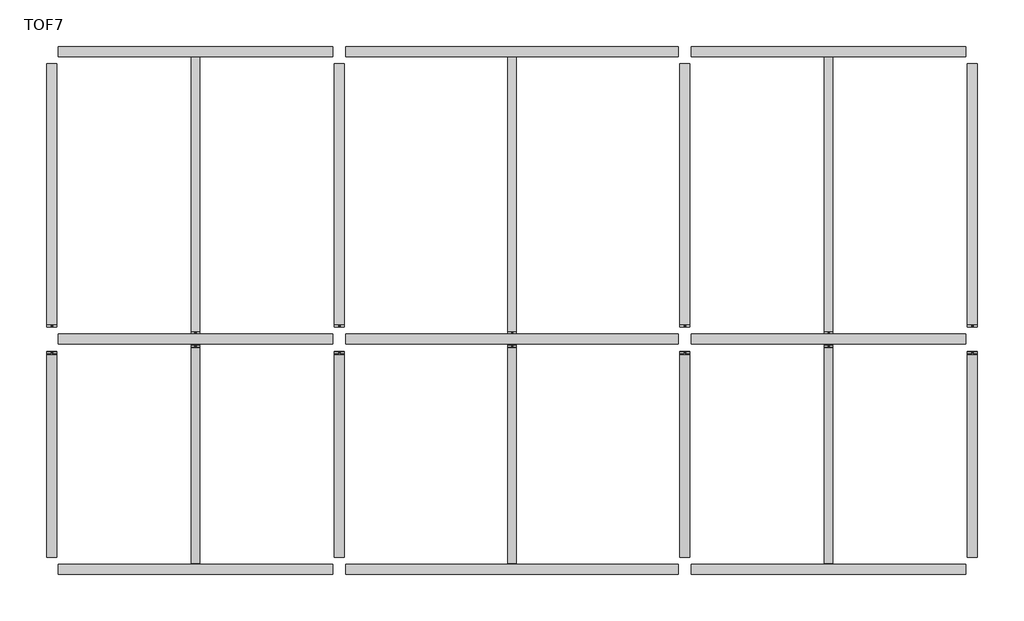
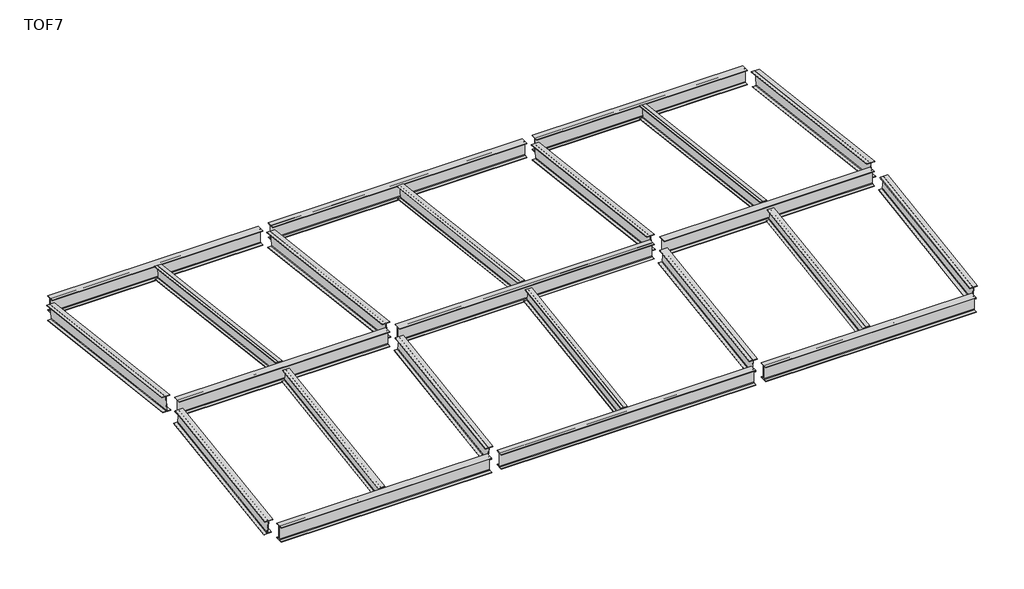
# One storey: 23 beams.
"""IFC4 building model written with IfcOpenShell, lengths in millimetres."""

import ifcopenshell
import ifcopenshell.guid

model = None  # the IFC model being written
_history = None  # IfcOwnerHistory: only IFC2X3 demands one
_inside = {}  # id of a spatial element -> (the spatial element, [elements in it])
_under = {}  # id of a project, library or spatial element -> (it, [spatial elements below it])
_declared = {}  # id of a project -> (the project, [libraries it declares])
_typed = {}  # id of a type object -> (the type object, [elements of that type])
_made_of = {}  # id of a material, layer set ... -> (it, [elements and type objects made of it])


def new_model(schema):
    """Start an empty IFC model of exactly this schema.

    Asked for "IFC4X3", IfcOpenShell would pick the latest addendum, in which some entities
    have other attributes; the version numbers below select the first issue.
    IFC2X3 requires an IfcOwnerHistory on every rooted entity: one is made here for all.
    """
    global model, _history
    if schema == "IFC4X3":
        model = ifcopenshell.file(schema_version=(4, 3, 0, 0))
    else:
        model = ifcopenshell.file(schema=schema)
    _inside.clear()
    _under.clear()
    _declared.clear()
    _typed.clear()
    _made_of.clear()
    _history = None
    if model.schema == "IFC2X3":
        org = make("IfcOrganization", Name="unknown")
        user = make(
            "IfcPersonAndOrganization",
            ThePerson=make("IfcPerson", FamilyName="unknown"),
            TheOrganization=org,
        )
        app = make(
            "IfcApplication",
            ApplicationDeveloper=org,
            Version="unknown",
            ApplicationFullName="unknown",
            ApplicationIdentifier="unknown",
        )
        _history = make(
            "IfcOwnerHistory",
            OwningUser=user,
            OwningApplication=app,
            ChangeAction="ADDED",
            CreationDate=0,
        )
    return model


def make(cls, **values):
    """One entity of the class cls with the attributes given. An attribute that is None is left unset."""
    return model.create_entity(
        cls, **{name: value for name, value in values.items() if value is not None}
    )


def rooted(cls, **values):
    """An entity with a GlobalId (a new one), such as an element, a storey or a relation."""
    return make(cls, GlobalId=ifcopenshell.guid.new(), OwnerHistory=_history, **values)


def si_unit(unit_type, name, prefix=None):
    """IfcSIUnit, for example si_unit("LENGTHUNIT", "METRE", prefix="MILLI")."""
    return make("IfcSIUnit", UnitType=unit_type, Prefix=prefix, Name=name)


def assignment(units):
    """IfcUnitAssignment: the units of a project."""
    return None if units is None else make("IfcUnitAssignment", Units=units)


def point(xyz):
    """IfcCartesianPoint."""
    return None if xyz is None else make("IfcCartesianPoint", Coordinates=xyz)


def direction(xyz):
    """IfcDirection."""
    return None if xyz is None else make("IfcDirection", DirectionRatios=xyz)


def frame(location, z_axis=None, x_axis=None):
    """IfcAxis2Placement3D, a coordinate frame: its origin and axes. An axis left out is left unset."""
    return make(
        "IfcAxis2Placement3D",
        Location=point(location),
        Axis=direction(z_axis),
        RefDirection=direction(x_axis),
    )


def frame_2d(location, x_axis=None):
    """IfcAxis2Placement2D, a coordinate frame in the plane: its origin and x axis."""
    return make(
        "IfcAxis2Placement2D", Location=point(location), RefDirection=direction(x_axis)
    )


def origin():
    """The frame at (0, 0, 0) with its axes left unset."""
    return frame((0.0, 0.0, 0.0))


def place(relative_to, where):
    """IfcLocalPlacement: puts the frame where relative to a parent placement (None: the world)."""
    return make(
        "IfcLocalPlacement", PlacementRelTo=relative_to, RelativePlacement=where
    )


def context(
    kind, dimensions, precision=None, world=None, true_north=None, identifier=None
):
    """IfcGeometricRepresentationContext, for example the 3D "Model" context."""
    return make(
        "IfcGeometricRepresentationContext",
        ContextIdentifier=identifier,
        ContextType=kind,
        CoordinateSpaceDimension=dimensions,
        Precision=precision,
        WorldCoordinateSystem=world,
        TrueNorth=true_north,
    )


def project(units=None, contexts=None):
    """IfcProject with its units and contexts."""
    return rooted(
        "IfcProject",
        Name="project",
        RepresentationContexts=contexts,
        UnitsInContext=assignment(units),
    )


def spatial(cls, under=None, at=None, **own):
    """A site, building, storey or space (cls), placed at a placement, below another one or the project."""
    s = rooted(cls, ObjectPlacement=at, **own)
    if under is not None:
        _under.setdefault(under.id(), (under, []))[1].append(s)
    return s


def polyline(points):
    """IfcPolyline through the points."""
    return make("IfcPolyline", Points=[point(p) for p in points])


def circle_curve(where, radius):
    """IfcCircle in the frame where."""
    return make("IfcCircle", Position=where, Radius=radius)


def trimmed(basis, trim1, trim2, sense, master):
    """IfcTrimmedCurve: the piece of a basis curve between two trims."""
    return make(
        "IfcTrimmedCurve",
        BasisCurve=basis,
        Trim1=trim1,
        Trim2=trim2,
        SenseAgreement=sense,
        MasterRepresentation=master,
    )


def segment(curve, same_sense, transition):
    """IfcCompositeCurveSegment."""
    return make(
        "IfcCompositeCurveSegment",
        Transition=transition,
        SameSense=same_sense,
        ParentCurve=curve,
    )


def composite_curve(segments, self_intersect=None):
    """IfcCompositeCurve: segments joined end to end."""
    return make("IfcCompositeCurve", Segments=segments, SelfIntersect=self_intersect)


def outline(outer, holes=None, kind="AREA"):
    """IfcArbitraryClosedProfileDef: a profile drawn as a closed curve; with holes, ...WithVoids."""
    if holes is None:
        return make("IfcArbitraryClosedProfileDef", ProfileType=kind, OuterCurve=outer)
    return make(
        "IfcArbitraryProfileDefWithVoids",
        ProfileType=kind,
        OuterCurve=outer,
        InnerCurves=holes,
    )


def extrude(swept, where, along, depth):
    """IfcExtrudedAreaSolid: the profile swept, set in the frame where, extruded along a direction by depth."""
    return make(
        "IfcExtrudedAreaSolid",
        SweptArea=swept,
        Position=where,
        ExtrudedDirection=direction(along),
        Depth=depth,
    )


def shape(context_of_items, identifier, shape_type, items):
    """IfcShapeRepresentation: the items that make up one representation, for example the "Body"."""
    return make(
        "IfcShapeRepresentation",
        ContextOfItems=context_of_items,
        RepresentationIdentifier=identifier,
        RepresentationType=shape_type,
        Items=items,
    )


def source(mapping_origin, context_of_items, identifier, shape_type, items):
    """IfcRepresentationMap: a shape defined once, which mapped items show again and again."""
    return make(
        "IfcRepresentationMap",
        MappingOrigin=mapping_origin,
        MappedRepresentation=shape(context_of_items, identifier, shape_type, items),
    )


def transform(
    local_origin,
    x_axis=None,
    y_axis=None,
    z_axis=None,
    scale=None,
    scale2=None,
    scale3=None,
    uniform=True,
):
    """IfcCartesianTransformationOperator3D, or its non-uniform kind. x_axis, y_axis, z_axis: its Axis1, 2, 3."""
    if uniform:
        return make(
            "IfcCartesianTransformationOperator3D",
            Axis1=direction(x_axis),
            Axis2=direction(y_axis),
            LocalOrigin=point(local_origin),
            Scale=scale,
            Axis3=direction(z_axis),
        )
    return make(
        "IfcCartesianTransformationOperator3DnonUniform",
        Axis1=direction(x_axis),
        Axis2=direction(y_axis),
        LocalOrigin=point(local_origin),
        Scale=scale,
        Axis3=direction(z_axis),
        Scale2=scale2,
        Scale3=scale3,
    )


def mapped(mapping_source, mapping_target):
    """IfcMappedItem: shows the shape of a source again, moved by a transform."""
    return make(
        "IfcMappedItem", MappingSource=mapping_source, MappingTarget=mapping_target
    )


def made_of(thing, what):
    """Note that an element or type object is made of a material, layer set ...; save() writes the relation."""
    if what is not None:
        _made_of.setdefault(what.id(), (what, []))[1].append(thing)
    return thing


def element(
    cls,
    number,
    at=None,
    inside=None,
    cuts=None,
    type_object=None,
    material=None,
    context=None,
    identifier="Body",
    shape_type=None,
    held_by="IfcProductDefinitionShape",
    body=None,
    shapes=None,
    **own,
):
    """One element of the class cls, such as IfcWall. Its Tag is "e" and its number.

    at: its placement. inside: the storey or other place that contains it. cuts: it is an
    opening in that element (IfcRelVoidsElement). A single representation is given by context,
    identifier, shape_type and body (its items); several are given by shapes. held_by: the class
    of the entity that holds the representations. save() writes the other relations.
    """
    e = rooted(cls, Tag="e%d" % number, ObjectPlacement=at, **own)
    if body is not None:
        shapes = [shape(context, identifier, shape_type, body)]
    if shapes is not None:
        e.Representation = make(held_by, Representations=shapes)
    if inside is not None:
        _inside.setdefault(inside.id(), (inside, []))[1].append(e)
    if cuts is not None:
        rooted(
            "IfcRelVoidsElement", RelatingBuildingElement=cuts, RelatedOpeningElement=e
        )
    if type_object is not None:
        _typed.setdefault(type_object.id(), (type_object, []))[1].append(e)
    return made_of(e, material)


def aggregate(whole, parts):
    """IfcRelAggregates: a whole, such as a stair, and the parts it consists of."""
    return rooted("IfcRelAggregates", RelatingObject=whole, RelatedObjects=parts)


def save(model, path):
    """Write the relations noted so far, then the file.

    IfcRelAggregates (storeys below a building ...), IfcRelContainedInSpatialStructure (elements
    in a storey), IfcRelDefinesByType, IfcRelAssociatesMaterial and IfcRelDeclares: one each for
    every whole, place, type object, material and project.
    """
    for whole, parts in _under.values():
        aggregate(whole, parts)
    for where, things in _inside.values():
        rooted(
            "IfcRelContainedInSpatialStructure",
            RelatedElements=things,
            RelatingStructure=where,
        )
    for kind, things in _typed.values():
        rooted("IfcRelDefinesByType", RelatedObjects=things, RelatingType=kind)
    for what, things in _made_of.values():
        rooted("IfcRelAssociatesMaterial", RelatedObjects=things, RelatingMaterial=what)
    for by, libraries in _declared.values():
        rooted("IfcRelDeclares", RelatingContext=by, RelatedDefinitions=libraries)
    model.write(path)


def beam_c38fbaf3(model_context):
    return source(origin(), model_context, "Body", "SweptSolid", [
        extrude(outline(composite_curve([segment(polyline([(75.0, -141.0), (75.0, -150.0), (-75.0, -150.0), (-75.0, -141.0), (-16.25, -141.0)]), True, "CONTINUOUS"), segment(trimmed(circle_curve(frame_2d((-16.25, -128.0)), 13.0), [point((-16.25, -141.0))], [point((-3.25, -128.0))], True, "CARTESIAN"), True, "CONTINUOUS"), segment(polyline([(-3.25, -128.0), (-3.25, 128.0)]), True, "CONTINUOUS"), segment(trimmed(circle_curve(frame_2d((-16.25, 128.0)), 13.0), [point((-3.25, 128.0))], [point((-16.25, 141.0))], True, "CARTESIAN"), True, "CONTINUOUS"), segment(polyline([(-16.25, 141.0), (-75.0, 141.0), (-75.0, 150.0), (75.0, 150.0), (75.0, 141.0), (16.25, 141.0)]), True, "CONTINUOUS"), segment(trimmed(circle_curve(frame_2d((16.25, 128.0)), 13.0), [point((16.25, 141.0))], [point((3.25, 128.0))], True, "CARTESIAN"), True, "CONTINUOUS"), segment(polyline([(3.25, 128.0), (3.25, -128.0)]), True, "CONTINUOUS"), segment(trimmed(circle_curve(frame_2d((16.25, -128.0)), 13.0), [point((3.25, -128.0))], [point((16.25, -141.0))], True, "CARTESIAN"), True, "CONTINUOUS"), segment(polyline([(16.25, -141.0), (75.0, -141.0)]), True, "CONTINUOUS")], self_intersect=False)), frame((-1923.1429107, 0.0, 0.0), z_axis=(1.0, 0.0, 0.0), x_axis=(0.0, 1.0, 0.0)), (0.0, 0.0, 1.0), 3799.338853),
    ])


def beam_fed367b4(model_context):
    return source(origin(), model_context, "Body", "SweptSolid", [
        extrude(outline(composite_curve([segment(polyline([(75.0, -141.0), (75.0, -150.0), (-75.0, -150.0), (-75.0, -141.0), (-16.25, -141.0)]), True, "CONTINUOUS"), segment(trimmed(circle_curve(frame_2d((-16.25, -128.0)), 13.0), [point((-16.25, -141.0))], [point((-3.25, -128.0))], True, "CARTESIAN"), True, "CONTINUOUS"), segment(polyline([(-3.25, -128.0), (-3.25, 128.0)]), True, "CONTINUOUS"), segment(trimmed(circle_curve(frame_2d((-16.25, 128.0)), 13.0), [point((-3.25, 128.0))], [point((-16.25, 141.0))], True, "CARTESIAN"), True, "CONTINUOUS"), segment(polyline([(-16.25, 141.0), (-75.0, 141.0), (-75.0, 150.0), (75.0, 150.0), (75.0, 141.0), (16.25, 141.0)]), True, "CONTINUOUS"), segment(trimmed(circle_curve(frame_2d((16.25, 128.0)), 13.0), [point((16.25, 141.0))], [point((3.25, 128.0))], True, "CARTESIAN"), True, "CONTINUOUS"), segment(polyline([(3.25, 128.0), (3.25, -128.0)]), True, "CONTINUOUS"), segment(trimmed(circle_curve(frame_2d((16.25, -128.0)), 13.0), [point((3.25, -128.0))], [point((16.25, -141.0))], True, "CARTESIAN"), True, "CONTINUOUS"), segment(polyline([(16.25, -141.0), (75.0, -141.0)]), True, "CONTINUOUS")], self_intersect=False)), frame((-2381.1079142, 0.0, 0.0), z_axis=(1.0, 0.0, 0.0), x_axis=(0.0, 1.0, 0.0)), (0.0, 0.0, 1.0), 4799.4668533),
    ])


def beam_74d50635(model_context):
    return source(origin(), model_context, "Body", "SweptSolid", [
        extrude(outline(composite_curve([segment(polyline([(87.5, -164.0), (87.5, -175.0), (-87.5, -175.0), (-87.5, -164.0), (-17.5, -164.0)]), True, "CONTINUOUS"), segment(trimmed(circle_curve(frame_2d((-17.5, -150.0)), 14.0), [point((-17.5, -164.0))], [point((-3.5, -150.0))], True, "CARTESIAN"), True, "CONTINUOUS"), segment(polyline([(-3.5, -150.0), (-3.5, 150.0)]), True, "CONTINUOUS"), segment(trimmed(circle_curve(frame_2d((-17.5, 150.0)), 14.0), [point((-3.5, 150.0))], [point((-17.5, 164.0))], True, "CARTESIAN"), True, "CONTINUOUS"), segment(polyline([(-17.5, 164.0), (-87.5, 164.0), (-87.5, 175.0), (87.5, 175.0), (87.5, 164.0), (17.5, 164.0)]), True, "CONTINUOUS"), segment(trimmed(circle_curve(frame_2d((17.5, 150.0)), 14.0), [point((17.5, 164.0))], [point((3.5, 150.0))], True, "CARTESIAN"), True, "CONTINUOUS"), segment(polyline([(3.5, 150.0), (3.5, -150.0)]), True, "CONTINUOUS"), segment(trimmed(circle_curve(frame_2d((17.5, -150.0)), 14.0), [point((3.5, -150.0))], [point((17.5, -164.0))], True, "CARTESIAN"), True, "CONTINUOUS"), segment(polyline([(17.5, -164.0), (87.5, -164.0)]), True, "CONTINUOUS")], self_intersect=False)), frame((-2387.3, 0.0, 0.0), z_axis=(1.0, 0.0, 0.0), x_axis=(0.0, 1.0, 0.0)), (0.0, 0.0, 1.0), 4774.6),
    ])


def beam_3a5a8fac(model_context):
    return source(origin(), model_context, "Body", "SweptSolid", [
        extrude(outline(composite_curve([segment(polyline([(87.5, -164.0), (87.5, -175.0), (-87.5, -175.0), (-87.5, -164.0), (-17.5, -164.0)]), True, "CONTINUOUS"), segment(trimmed(circle_curve(frame_2d((-17.5, -150.0)), 14.0), [point((-17.5, -164.0))], [point((-3.5, -150.0))], True, "CARTESIAN"), True, "CONTINUOUS"), segment(polyline([(-3.5, -150.0), (-3.5, 150.0)]), True, "CONTINUOUS"), segment(trimmed(circle_curve(frame_2d((-17.5, 150.0)), 14.0), [point((-3.5, 150.0))], [point((-17.5, 164.0))], True, "CARTESIAN"), True, "CONTINUOUS"), segment(polyline([(-17.5, 164.0), (-87.5, 164.0), (-87.5, 175.0), (87.5, 175.0), (87.5, 164.0), (17.5, 164.0)]), True, "CONTINUOUS"), segment(trimmed(circle_curve(frame_2d((17.5, 150.0)), 14.0), [point((17.5, 164.0))], [point((3.5, 150.0))], True, "CARTESIAN"), True, "CONTINUOUS"), segment(polyline([(3.5, 150.0), (3.5, -150.0)]), True, "CONTINUOUS"), segment(trimmed(circle_curve(frame_2d((17.5, -150.0)), 14.0), [point((3.5, -150.0))], [point((17.5, -164.0))], True, "CARTESIAN"), True, "CONTINUOUS"), segment(polyline([(17.5, -164.0), (87.5, -164.0)]), True, "CONTINUOUS")], self_intersect=False)), frame((-2887.3, 0.0, 0.0), z_axis=(1.0, 0.0, 0.0), x_axis=(0.0, 1.0, 0.0)), (0.0, 0.0, 1.0), 5774.6),
    ])


def beam_9c24ba7d(model_context):
    return source(origin(), model_context, "Body", "SweptSolid", [
        extrude(outline(composite_curve([segment(polyline([(87.5, -164.0), (87.5, -175.0), (-87.5, -175.0), (-87.5, -164.0), (-17.5, -164.0)]), True, "CONTINUOUS"), segment(trimmed(circle_curve(frame_2d((-17.5, -150.0)), 14.0), [point((-17.5, -164.0))], [point((-3.5, -150.0))], True, "CARTESIAN"), True, "CONTINUOUS"), segment(polyline([(-3.5, -150.0), (-3.5, 150.0)]), True, "CONTINUOUS"), segment(trimmed(circle_curve(frame_2d((-17.5, 150.0)), 14.0), [point((-3.5, 150.0))], [point((-17.5, 164.0))], True, "CARTESIAN"), True, "CONTINUOUS"), segment(polyline([(-17.5, 164.0), (-87.5, 164.0), (-87.5, 175.0), (87.5, 175.0), (87.5, 164.0), (17.5, 164.0)]), True, "CONTINUOUS"), segment(trimmed(circle_curve(frame_2d((17.5, 150.0)), 14.0), [point((17.5, 164.0))], [point((3.5, 150.0))], True, "CARTESIAN"), True, "CONTINUOUS"), segment(polyline([(3.5, 150.0), (3.5, -150.0)]), True, "CONTINUOUS"), segment(trimmed(circle_curve(frame_2d((17.5, -150.0)), 14.0), [point((3.5, -150.0))], [point((17.5, -164.0))], True, "CARTESIAN"), True, "CONTINUOUS"), segment(polyline([(17.5, -164.0), (87.5, -164.0)]), True, "CONTINUOUS")], self_intersect=False)), frame((-1811.887571, 0.0, 0.0), z_axis=(1.0, 0.0, 0.0), x_axis=(0.0, 1.0, 0.0)), (0.0, 0.0, 1.0), 3566.8249285),
    ])


def beam_94df1702(model_context):
    return source(origin(), model_context, "Body", "SweptSolid", [
        extrude(outline(composite_curve([segment(polyline([(87.5, -164.0), (87.5, -175.0), (-87.5, -175.0), (-87.5, -164.0), (-17.5, -164.0)]), True, "CONTINUOUS"), segment(trimmed(circle_curve(frame_2d((-17.5, -150.0)), 14.0), [point((-17.5, -164.0))], [point((-3.5, -150.0))], True, "CARTESIAN"), True, "CONTINUOUS"), segment(polyline([(-3.5, -150.0), (-3.5, 150.0)]), True, "CONTINUOUS"), segment(trimmed(circle_curve(frame_2d((-17.5, 150.0)), 14.0), [point((-3.5, 150.0))], [point((-17.5, 164.0))], True, "CARTESIAN"), True, "CONTINUOUS"), segment(polyline([(-17.5, 164.0), (-87.5, 164.0), (-87.5, 175.0), (87.5, 175.0), (87.5, 164.0), (17.5, 164.0)]), True, "CONTINUOUS"), segment(trimmed(circle_curve(frame_2d((17.5, 150.0)), 14.0), [point((17.5, 164.0))], [point((3.5, 150.0))], True, "CARTESIAN"), True, "CONTINUOUS"), segment(polyline([(3.5, 150.0), (3.5, -150.0)]), True, "CONTINUOUS"), segment(trimmed(circle_curve(frame_2d((17.5, -150.0)), 14.0), [point((3.5, -150.0))], [point((17.5, -164.0))], True, "CARTESIAN"), True, "CONTINUOUS"), segment(polyline([(17.5, -164.0), (87.5, -164.0)]), True, "CONTINUOUS")], self_intersect=False)), frame((-2261.8008094, 0.0, 0.0), z_axis=(1.0, 0.0, 0.0), x_axis=(0.0, 1.0, 0.0)), (0.0, 0.0, 1.0), 4568.4611041),
    ])


model = new_model("IFC4")

# Units and contexts
model_context = context("Model", 3, world=origin())
ifc_project = project(units=[si_unit("LENGTHUNIT", "METRE", prefix="MILLI")], contexts=[model_context])

# Site, building, storey
site = spatial("IfcSite", under=ifc_project)
building = spatial("IfcBuilding", under=site)
storey = spatial("IfcBuildingStorey", under=building, Name="TOF7", Elevation=12500.0)

# Beams
placement = place(None, origin())
beam_shape = beam_c38fbaf3(model_context)
element("IfcBeam", 1, ObjectType="0912_Steel Framing_H-KSD3502 : H_SB_AR_S02_H-300x150x6.5x9_Stair", at=placement, inside=storey, context=model_context, shape_type="MappedRepresentation", body=[
    mapped(beam_shape, transform((2500.0, 2022.2510679, 12651.6595471), x_axis=(0.0, 0.9889363528682974, 0.14834045293024514), y_axis=(-1.0, 0.0, 0.0), z_axis=(0.0, -0.14834045293024517, 0.9889363528682975))),
])
element("IfcBeam", 2, ObjectType="0912_Steel Framing_H-KSD3502 : H_SB_AR_S02_H-300x150x6.5x9_Stair", at=placement, inside=storey, context=model_context, shape_type="MappedRepresentation", body=[
    mapped(beam_shape, transform((8000.0, 2022.2510679, 12651.6595471), x_axis=(0.0, 0.9889363528682974, 0.14834045293024514), y_axis=(-1.0, 0.0, 0.0), z_axis=(0.0, -0.14834045293024517, 0.9889363528682975))),
])
element("IfcBeam", 3, ObjectType="0912_Steel Framing_H-KSD3502 : H_SB_AR_S02_H-300x150x6.5x9_Stair", at=placement, inside=storey, context=model_context, shape_type="MappedRepresentation", body=[
    mapped(beam_shape, transform((13500.0, 2022.2510679, 12651.6595471), x_axis=(0.0, 0.9889363528682974, 0.14834045293024514), y_axis=(-1.0, 0.0, 0.0), z_axis=(0.0, -0.14834045293024517, 0.9889363528682975))),
])
beam_2_shape = beam_fed367b4(model_context)
element("IfcBeam", 4, ObjectType="0912_Steel Framing_H-KSD3502 : H_SB_AR_S02_H-300x150x6.5x9_Stair", at=placement, inside=storey, context=model_context, shape_type="MappedRepresentation", body=[
    mapped(beam_2_shape, transform((2500.0, 6482.1282169, 12651.0684742), x_axis=(0.0, 0.992876838486922, -0.11914522061843061), y_axis=(-1.0, 0.0, 0.0), z_axis=(0.0, 0.11914522061843062, 0.9928768384869221))),
])
element("IfcBeam", 5, ObjectType="0912_Steel Framing_H-KSD3502 : H_SB_AR_S02_H-300x150x6.5x9_Stair", at=placement, inside=storey, context=model_context, shape_type="MappedRepresentation", body=[
    mapped(beam_2_shape, transform((8000.0, 6482.1282169, 12651.0684742), x_axis=(0.0, 0.992876838486922, -0.11914522061843061), y_axis=(-1.0, 0.0, 0.0), z_axis=(0.0, 0.11914522061843062, 0.9928768384869221))),
])
element("IfcBeam", 6, ObjectType="0912_Steel Framing_H-KSD3502 : H_SB_AR_S02_H-300x150x6.5x9_Stair", at=placement, inside=storey, context=model_context, shape_type="MappedRepresentation", body=[
    mapped(beam_2_shape, transform((13500.0, 6482.1282169, 12651.0684742), x_axis=(0.0, 0.992876838486922, -0.11914522061843061), y_axis=(-1.0, 0.0, 0.0), z_axis=(0.0, 0.11914522061843062, 0.9928768384869221))),
])
beam_3_shape = beam_74d50635(model_context)
element("IfcBeam", 7, ObjectType="0912_Steel Framing_H-KSD3502 : H_SB_AR_S02_H-350x175x7x11_Platform", at=placement, inside=storey, context=model_context, shape_type="MappedRepresentation", body=[
    mapped(beam_3_shape, transform((2500.0, 0.0, 12325.0), x_axis=(1.0, 0.0, 0.0), y_axis=(0.0, 1.0, 0.0), z_axis=(0.0, 0.0, 1.0))),
])
element("IfcBeam", 8, ObjectType="0912_Steel Framing_H-KSD3502 : H_SB_AR_S02_H-350x175x7x11_Platform", at=placement, inside=storey, context=model_context, shape_type="MappedRepresentation", body=[
    mapped(beam_3_shape, transform((13500.0, 0.0, 12325.0), x_axis=(1.0, 0.0, 0.0), y_axis=(0.0, 1.0, 0.0), z_axis=(0.0, 0.0, 1.0))),
])
element("IfcBeam", 9, ObjectType="0912_Steel Framing_H-KSD3502 : H_SB_AR_S02_H-350x175x7x11_Platform", at=placement, inside=storey, context=model_context, shape_type="MappedRepresentation", body=[
    mapped(beam_3_shape, transform((2500.0, 4000.0, 12925.0), x_axis=(1.0, 0.0, 0.0), y_axis=(0.0, 1.0, 0.0), z_axis=(0.0, 0.0, 1.0))),
])
element("IfcBeam", 10, ObjectType="0912_Steel Framing_H-KSD3502 : H_SB_AR_S02_H-350x175x7x11_Platform", at=placement, inside=storey, context=model_context, shape_type="MappedRepresentation", body=[
    mapped(beam_3_shape, transform((13500.0, 4000.0, 12925.0), x_axis=(1.0, 0.0, 0.0), y_axis=(0.0, 1.0, 0.0), z_axis=(0.0, 0.0, 1.0))),
])
element("IfcBeam", 11, ObjectType="0912_Steel Framing_H-KSD3502 : H_SB_AR_S02_H-350x175x7x11_Platform", at=placement, inside=storey, context=model_context, shape_type="MappedRepresentation", body=[
    mapped(beam_3_shape, transform((2500.0, 9000.0, 12325.0), x_axis=(1.0, 0.0, 0.0), y_axis=(0.0, 1.0, 0.0), z_axis=(0.0, 0.0, 1.0))),
])
element("IfcBeam", 12, ObjectType="0912_Steel Framing_H-KSD3502 : H_SB_AR_S02_H-350x175x7x11_Platform", at=placement, inside=storey, context=model_context, shape_type="MappedRepresentation", body=[
    mapped(beam_3_shape, transform((13500.0, 9000.0, 12325.0), x_axis=(1.0, 0.0, 0.0), y_axis=(0.0, 1.0, 0.0), z_axis=(0.0, 0.0, 1.0))),
])
beam_4_shape = beam_3a5a8fac(model_context)
element("IfcBeam", 13, ObjectType="0912_Steel Framing_H-KSD3502 : H_SB_AR_S02_H-350x175x7x11_Platform", at=placement, inside=storey, context=model_context, shape_type="MappedRepresentation", body=[
    mapped(beam_4_shape, transform((8000.0, 0.0, 12325.0), x_axis=(1.0, 0.0, 0.0), y_axis=(0.0, 1.0, 0.0), z_axis=(0.0, 0.0, 1.0))),
])
element("IfcBeam", 14, ObjectType="0912_Steel Framing_H-KSD3502 : H_SB_AR_S02_H-350x175x7x11_Platform", at=placement, inside=storey, context=model_context, shape_type="MappedRepresentation", body=[
    mapped(beam_4_shape, transform((8000.0, 4000.0, 12925.0), x_axis=(1.0, 0.0, 0.0), y_axis=(0.0, 1.0, 0.0), z_axis=(0.0, 0.0, 1.0))),
])
element("IfcBeam", 15, ObjectType="0912_Steel Framing_H-KSD3502 : H_SB_AR_S02_H-350x175x7x11_Platform", at=placement, inside=storey, context=model_context, shape_type="MappedRepresentation", body=[
    mapped(beam_4_shape, transform((8000.0, 9000.0, 12325.0), x_axis=(1.0, 0.0, 0.0), y_axis=(0.0, 1.0, 0.0), z_axis=(0.0, 0.0, 1.0))),
])
beam_5_shape = beam_9c24ba7d(model_context)
element("IfcBeam", 16, ObjectType="0912_Steel Framing_H-KSD3502 : H_SB_AR_S02_H-350x175x7x11_Platform", at=placement, inside=storey, context=model_context, shape_type="MappedRepresentation", body=[
    mapped(beam_5_shape, transform((0.0, 2025.9595793, 12626.9361382), x_axis=(0.0, 0.9889363528682974, 0.14834045293024514), y_axis=(-1.0, 0.0, 0.0), z_axis=(0.0, -0.14834045293024517, 0.9889363528682975))),
])
element("IfcBeam", 17, ObjectType="0912_Steel Framing_H-KSD3502 : H_SB_AR_S02_H-350x175x7x11_Platform", at=placement, inside=storey, context=model_context, shape_type="MappedRepresentation", body=[
    mapped(beam_5_shape, transform((5000.0, 2025.9595793, 12626.9361382), x_axis=(0.0, 0.9889363528682974, 0.14834045293024514), y_axis=(-1.0, 0.0, 0.0), z_axis=(0.0, -0.14834045293024517, 0.9889363528682975))),
])
element("IfcBeam", 18, ObjectType="0912_Steel Framing_H-KSD3502 : H_SB_AR_S02_H-350x175x7x11_Platform", at=placement, inside=storey, context=model_context, shape_type="MappedRepresentation", body=[
    mapped(beam_5_shape, transform((11000.0, 2025.9595793, 12626.9361382), x_axis=(0.0, 0.9889363528682974, 0.14834045293024514), y_axis=(-1.0, 0.0, 0.0), z_axis=(0.0, -0.14834045293024517, 0.9889363528682975))),
])
element("IfcBeam", 19, ObjectType="0912_Steel Framing_H-KSD3502 : H_SB_AR_S02_H-350x175x7x11_Platform", at=placement, inside=storey, context=model_context, shape_type="MappedRepresentation", body=[
    mapped(beam_5_shape, transform((16000.0, 2025.9595793, 12626.9361382), x_axis=(0.0, 0.9889363528682974, 0.14834045293024514), y_axis=(-1.0, 0.0, 0.0), z_axis=(0.0, -0.14834045293024517, 0.9889363528682975))),
])
beam_6_shape = beam_94df1702(model_context)
element("IfcBeam", 20, ObjectType="0912_Steel Framing_H-KSD3502 : H_SB_AR_S02_H-350x175x7x11_Platform", at=placement, inside=storey, context=model_context, shape_type="MappedRepresentation", body=[
    mapped(beam_6_shape, transform((0.0, 6479.1495864, 12626.2465533), x_axis=(0.0, 0.992876838486922, -0.11914522061843061), y_axis=(-1.0, 0.0, 0.0), z_axis=(0.0, 0.11914522061843065, 0.9928768384869221))),
])
element("IfcBeam", 21, ObjectType="0912_Steel Framing_H-KSD3502 : H_SB_AR_S02_H-350x175x7x11_Platform", at=placement, inside=storey, context=model_context, shape_type="MappedRepresentation", body=[
    mapped(beam_6_shape, transform((5000.0, 6479.1495864, 12626.2465533), x_axis=(0.0, 0.992876838486922, -0.11914522061843061), y_axis=(-1.0, 0.0, 0.0), z_axis=(0.0, 0.11914522061843065, 0.9928768384869221))),
])
element("IfcBeam", 22, ObjectType="0912_Steel Framing_H-KSD3502 : H_SB_AR_S02_H-350x175x7x11_Platform", at=placement, inside=storey, context=model_context, shape_type="MappedRepresentation", body=[
    mapped(beam_6_shape, transform((11000.0, 6479.1495864, 12626.2465533), x_axis=(0.0, 0.992876838486922, -0.11914522061843061), y_axis=(-1.0, 0.0, 0.0), z_axis=(0.0, 0.11914522061843065, 0.9928768384869221))),
])
element("IfcBeam", 23, ObjectType="0912_Steel Framing_H-KSD3502 : H_SB_AR_S02_H-350x175x7x11_Platform", at=placement, inside=storey, context=model_context, shape_type="MappedRepresentation", body=[
    mapped(beam_6_shape, transform((16000.0, 6479.1495864, 12626.2465533), x_axis=(0.0, 0.992876838486922, -0.11914522061843061), y_axis=(-1.0, 0.0, 0.0), z_axis=(0.0, 0.11914522061843065, 0.9928768384869221))),
])

save(model, "model.ifc")

# Revit data of these elements
# Type "0912_Steel Framing_H-KSD3502 : H_SB_AR_S02_H-300x150x6.5x9_Stair"
#   H_Q'ty Cal Type Tag = "SB-Q2"
#   H_WM Code_1 = "S01AA073-00001 |  | TON | Main Steel Structure Fabrication Work | Shelter/Building | Medium Steel - Standard |  |  |  |  |  |  | Material: (   ) | (90)KG/M>Weight≥(30)KG/M | S01AA073-00001 Main Steel Structure Fabrication Work Shelter/Building Medium Steel - Standard         | - Material: ( ASTM A36 )\n- (90)KG/M>Weight≥(30)KG/M"
#   H_WM Code_2 = "S03AA083-00001 |  | TON | Main Steel Structure Erection Work | Shelter/Building | Medium Steel |  |  |  |  |  |  | Material: (   ) | S03AA083-00001 Main Steel Structure Erection Work Shelter/Building Medium Steel         | - Material: ( ASTM A36 )"
#   H_WM Code_3 = "S01AA009-00001 |  | TON | Main Steel Structure Fabrication Work | Shelter/Building | Plates - Gusset, Stiffener, ETC | Material: (   ) | S01AA009-00001 Main Steel Structure Fabrication Work Shelter/Building Plates - Gusset, Stiffener, ETC         |"
#   H_WM Code_4 = "S41AA051-00001 |  | M2 | Steel Structure Paint Work | Shelter/Building | for Non-Fireproofed Steel Surface |  |  |  |  |  |  | Material: (   ) | S41AA051-00001 Steel Structure Paint Work Shelter/Building for Non-Fireproofed Steel Surface         |"
#   Width = 15.0 cm
#   Web Thickness = 0.65 cm
#   Web Fillet = 1.3 cm
#   Warping Constant = 107000.0 cm⁶
#   W = 0
#   Torsional Moment of Inertia = 9.9539 cm⁴
#   Section Area = 46.78 cm²
#   Plastic Modulus weak axis = 105.0 cm³
#   Plastic Modulus strong axis = 542.0 cm³
#   Perimeter = 1.17 m²/m
#   Nominal Weight = 36.70 kgf/m
#   Moment of Inertia weak axis = 508.00 cm⁴
#   Moment of Inertia strong axis = 7210.00 cm⁴
#   Height = 30.0 cm
#   Flange Thickness = 0.9 cm
#   Elastic Modulus weak axis = 67.7 cm³
#   Elastic Modulus strong axis = 481.0 cm³
#   Centroid Vertical = 15.0 cm
#   Centroid Horizontal = 7.5 cm
#   Ix = 72100000
#   Length [instance default] = 1524 mm
#   Zx = 542000
#   b = 150 mm
#   h = 300 mm
#   r = 13 mm
#   s = 6.5 mm
#   t = 9 mm
#   A = 0.004678 m²
#   Structural Material [instance default] = Steel, 45-345
#   Assembly Code = ""
# Type "0912_Steel Framing_H-KSD3502 : H_SB_AR_S02_H-350x175x7x11_Platform"
#   H_Q'ty Cal Type Tag = "SB-Q2"
#   H_WM Code_1 = "S01AA073-00001 |  | TON | Main Steel Structure Fabrication Work | Shelter/Building | Medium Steel - Standard |  |  |  |  |  |  | Material: (   ) | (90)KG/M>Weight≥(30)KG/M | S01AA073-00001 Main Steel Structure Fabrication Work Shelter/Building Medium Steel - Standard         | - Material: ( ASTM A36 )\n- (90)KG/M>Weight≥(30)KG/M"
#   H_WM Code_2 = "S03AA083-00001 |  | TON | Main Steel Structure Erection Work | Shelter/Building | Medium Steel |  |  |  |  |  |  | Material: (   ) | S03AA083-00001 Main Steel Structure Erection Work Shelter/Building Medium Steel         | - Material: ( ASTM A36 )"
#   H_WM Code_3 = "S01AA009-00001 |  | TON | Main Steel Structure Fabrication Work | Shelter/Building | Plates - Gusset, Stiffener, ETC | Material: (   ) | S01AA009-00001 Main Steel Structure Fabrication Work Shelter/Building Plates - Gusset, Stiffener, ETC         |"
#   H_WM Code_4 = "S41AA051-00001 |  | M2 | Steel Structure Paint Work | Shelter/Building | for Non-Fireproofed Steel Surface |  |  |  |  |  |  | Material: (   ) | S41AA051-00001 Steel Structure Paint Work Shelter/Building for Non-Fireproofed Steel Surface         |"
#   Width = 17.5 cm
#   Web Thickness = 0.7 cm
#   Web Fillet = 1.4 cm
#   Warping Constant = 282000.0 cm⁶
#   W = 0
#   Torsional Moment of Inertia = 19.4042 cm⁴
#   Section Area = 63.14 cm²
#   Plastic Modulus weak axis = 174.0 cm³
#   Plastic Modulus strong axis = 868.0 cm³
#   Perimeter = 1.36 m²/m
#   Nominal Weight = 49.60 kgf/m
#   Moment of Inertia weak axis = 984.00 cm⁴
#   Moment of Inertia strong axis = 13600.00 cm⁴
#   Height = 35.0 cm
#   Flange Thickness = 1.1 cm
#   Elastic Modulus weak axis = 112.0 cm³
#   Elastic Modulus strong axis = 775.0 cm³
#   Centroid Vertical = 17.5 cm
#   Centroid Horizontal = 8.75 cm
#   Ix = 136000000
#   Length [instance default] = 1524 mm
#   Zx = 868000
#   b = 175 mm
#   h = 350 mm
#   r = 14 mm
#   s = 7 mm
#   t = 11 mm
#   A = 0.006314 m²
#   Structural Material [instance default] = Steel, 45-345
#   Assembly Code = ""
# Elements 1, 2, 3, 4, 5, 6 (IfcBeam, "0912_Steel Framing_H-KSD3502 : H_SB_AR_S02_H-300x150x6.5x9_Stair")
#   Comments = ""
#   Structural Material = Steel, 45-345
#   Phase Created = New Construction
#   Materials on its faces: "Steel, 45-345"
# Elements 7, 8, 9, 10, 11, 12, 13, 14, 15, 16, 17, 18, 19, 20, 21, 22, 23 (IfcBeam, "0912_Steel Framing_H-KSD3502 : H_SB_AR_S02_H-350x175x7x11_Platform")
#   Comments = ""
#   Structural Material = Steel, 45-345
#   Phase Created = New Construction
#   Materials on its faces: "Steel, 45-345"
# Materials
#   "Steel, 45-345": class "Metal", colour RGB 189 187 185, transparency 0, Description = "Steel 345 MPa", Cost = 0
